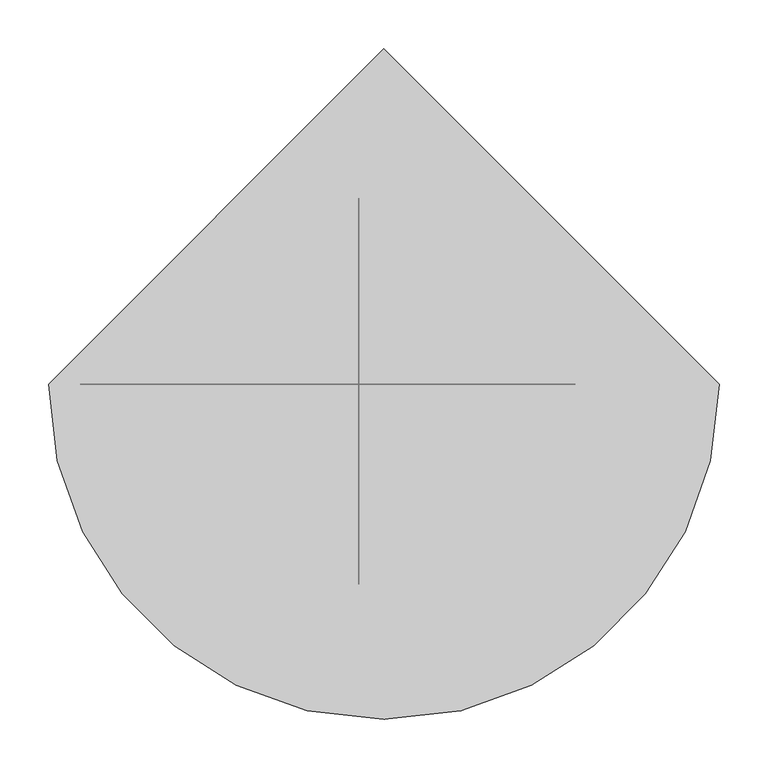
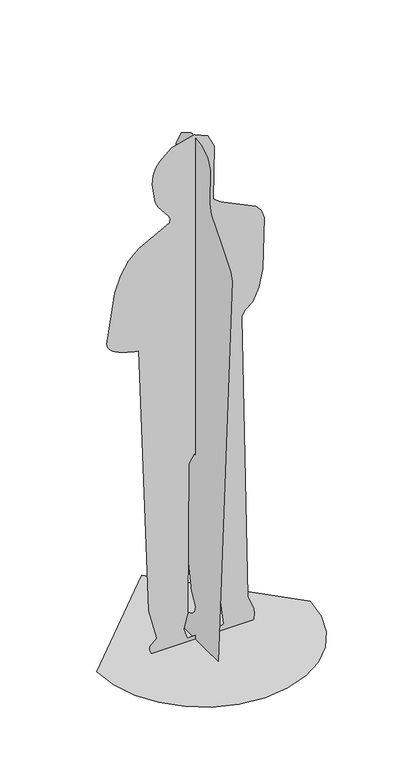
"""IFC4 building model written with IfcOpenShell, lengths in millimetres: proxy geometry, jay 23630 : jay 23630."""

import ifcopenshell
import ifcopenshell.guid

model = None  # the IFC model being written
_history = None  # IfcOwnerHistory: only IFC2X3 demands one
_inside = {}  # id of a spatial element -> (the spatial element, [elements in it])
_under = {}  # id of a project, library or spatial element -> (it, [spatial elements below it])
_declared = {}  # id of a project -> (the project, [libraries it declares])
_typed = {}  # id of a type object -> (the type object, [elements of that type])
_made_of = {}  # id of a material, layer set ... -> (it, [elements and type objects made of it])


def new_model(schema):
    """Start an empty IFC model of exactly this schema.

    Asked for "IFC4X3", IfcOpenShell would pick the latest addendum, in which some entities
    have other attributes; the version numbers below select the first issue.
    IFC2X3 requires an IfcOwnerHistory on every rooted entity: one is made here for all.
    """
    global model, _history
    if schema == "IFC4X3":
        model = ifcopenshell.file(schema_version=(4, 3, 0, 0))
    else:
        model = ifcopenshell.file(schema=schema)
    _inside.clear()
    _under.clear()
    _declared.clear()
    _typed.clear()
    _made_of.clear()
    _history = None
    if model.schema == "IFC2X3":
        org = make("IfcOrganization", Name="unknown")
        user = make(
            "IfcPersonAndOrganization",
            ThePerson=make("IfcPerson", FamilyName="unknown"),
            TheOrganization=org,
        )
        app = make(
            "IfcApplication",
            ApplicationDeveloper=org,
            Version="unknown",
            ApplicationFullName="unknown",
            ApplicationIdentifier="unknown",
        )
        _history = make(
            "IfcOwnerHistory",
            OwningUser=user,
            OwningApplication=app,
            ChangeAction="ADDED",
            CreationDate=0,
        )
    return model


def make(cls, **values):
    """One entity of the class cls with the attributes given. An attribute that is None is left unset."""
    return model.create_entity(
        cls, **{name: value for name, value in values.items() if value is not None}
    )


def rooted(cls, **values):
    """An entity with a GlobalId (a new one), such as an element, a storey or a relation."""
    return make(cls, GlobalId=ifcopenshell.guid.new(), OwnerHistory=_history, **values)


def si_unit(unit_type, name, prefix=None):
    """IfcSIUnit, for example si_unit("LENGTHUNIT", "METRE", prefix="MILLI")."""
    return make("IfcSIUnit", UnitType=unit_type, Prefix=prefix, Name=name)


def assignment(units):
    """IfcUnitAssignment: the units of a project."""
    return None if units is None else make("IfcUnitAssignment", Units=units)


def point(xyz):
    """IfcCartesianPoint."""
    return None if xyz is None else make("IfcCartesianPoint", Coordinates=xyz)


def direction(xyz):
    """IfcDirection."""
    return None if xyz is None else make("IfcDirection", DirectionRatios=xyz)


def frame(location, z_axis=None, x_axis=None):
    """IfcAxis2Placement3D, a coordinate frame: its origin and axes. An axis left out is left unset."""
    return make(
        "IfcAxis2Placement3D",
        Location=point(location),
        Axis=direction(z_axis),
        RefDirection=direction(x_axis),
    )


def origin():
    """The frame at (0, 0, 0) with its axes left unset."""
    return frame((0.0, 0.0, 0.0))


def place(relative_to, where):
    """IfcLocalPlacement: puts the frame where relative to a parent placement (None: the world)."""
    return make(
        "IfcLocalPlacement", PlacementRelTo=relative_to, RelativePlacement=where
    )


def context(
    kind, dimensions, precision=None, world=None, true_north=None, identifier=None
):
    """IfcGeometricRepresentationContext, for example the 3D "Model" context."""
    return make(
        "IfcGeometricRepresentationContext",
        ContextIdentifier=identifier,
        ContextType=kind,
        CoordinateSpaceDimension=dimensions,
        Precision=precision,
        WorldCoordinateSystem=world,
        TrueNorth=true_north,
    )


def project(units=None, contexts=None):
    """IfcProject with its units and contexts."""
    return rooted(
        "IfcProject",
        Name="project",
        RepresentationContexts=contexts,
        UnitsInContext=assignment(units),
    )


def spatial(cls, under=None, at=None, **own):
    """A site, building, storey or space (cls), placed at a placement, below another one or the project."""
    s = rooted(cls, ObjectPlacement=at, **own)
    if under is not None:
        _under.setdefault(under.id(), (under, []))[1].append(s)
    return s


def point_list(points):
    """IfcCartesianPointList2D or 3D."""
    cls = (
        "IfcCartesianPointList2D" if len(points[0]) == 2 else "IfcCartesianPointList3D"
    )
    return make(cls, CoordList=points)


def triangles(points, corners, closed=None, point_numbers=None):
    """IfcTriangulatedFaceSet: each triangle names its three corners, points numbered from 1."""
    return make(
        "IfcTriangulatedFaceSet",
        Coordinates=point_list(points),
        Closed=closed,
        CoordIndex=corners,
        PnIndex=point_numbers,
    )


def shape(context_of_items, identifier, shape_type, items):
    """IfcShapeRepresentation: the items that make up one representation, for example the "Body"."""
    return make(
        "IfcShapeRepresentation",
        ContextOfItems=context_of_items,
        RepresentationIdentifier=identifier,
        RepresentationType=shape_type,
        Items=items,
    )


def source(mapping_origin, context_of_items, identifier, shape_type, items):
    """IfcRepresentationMap: a shape defined once, which mapped items show again and again."""
    return make(
        "IfcRepresentationMap",
        MappingOrigin=mapping_origin,
        MappedRepresentation=shape(context_of_items, identifier, shape_type, items),
    )


def transform(
    local_origin,
    x_axis=None,
    y_axis=None,
    z_axis=None,
    scale=None,
    scale2=None,
    scale3=None,
    uniform=True,
):
    """IfcCartesianTransformationOperator3D, or its non-uniform kind. x_axis, y_axis, z_axis: its Axis1, 2, 3."""
    if uniform:
        return make(
            "IfcCartesianTransformationOperator3D",
            Axis1=direction(x_axis),
            Axis2=direction(y_axis),
            LocalOrigin=point(local_origin),
            Scale=scale,
            Axis3=direction(z_axis),
        )
    return make(
        "IfcCartesianTransformationOperator3DnonUniform",
        Axis1=direction(x_axis),
        Axis2=direction(y_axis),
        LocalOrigin=point(local_origin),
        Scale=scale,
        Axis3=direction(z_axis),
        Scale2=scale2,
        Scale3=scale3,
    )


def mapped(mapping_source, mapping_target):
    """IfcMappedItem: shows the shape of a source again, moved by a transform."""
    return make(
        "IfcMappedItem", MappingSource=mapping_source, MappingTarget=mapping_target
    )


def made_of(thing, what):
    """Note that an element or type object is made of a material, layer set ...; save() writes the relation."""
    if what is not None:
        _made_of.setdefault(what.id(), (what, []))[1].append(thing)
    return thing


def element(
    cls,
    number,
    at=None,
    inside=None,
    cuts=None,
    type_object=None,
    material=None,
    context=None,
    identifier="Body",
    shape_type=None,
    held_by="IfcProductDefinitionShape",
    body=None,
    shapes=None,
    **own,
):
    """One element of the class cls, such as IfcWall. Its Tag is "e" and its number.

    at: its placement. inside: the storey or other place that contains it. cuts: it is an
    opening in that element (IfcRelVoidsElement). A single representation is given by context,
    identifier, shape_type and body (its items); several are given by shapes. held_by: the class
    of the entity that holds the representations. save() writes the other relations.
    """
    e = rooted(cls, Tag="e%d" % number, ObjectPlacement=at, **own)
    if body is not None:
        shapes = [shape(context, identifier, shape_type, body)]
    if shapes is not None:
        e.Representation = make(held_by, Representations=shapes)
    if inside is not None:
        _inside.setdefault(inside.id(), (inside, []))[1].append(e)
    if cuts is not None:
        rooted(
            "IfcRelVoidsElement", RelatingBuildingElement=cuts, RelatedOpeningElement=e
        )
    if type_object is not None:
        _typed.setdefault(type_object.id(), (type_object, []))[1].append(e)
    return made_of(e, material)


def aggregate(whole, parts):
    """IfcRelAggregates: a whole, such as a stair, and the parts it consists of."""
    return rooted("IfcRelAggregates", RelatingObject=whole, RelatedObjects=parts)


def save(model, path):
    """Write the relations noted so far, then the file.

    IfcRelAggregates (storeys below a building ...), IfcRelContainedInSpatialStructure (elements
    in a storey), IfcRelDefinesByType, IfcRelAssociatesMaterial and IfcRelDeclares: one each for
    every whole, place, type object, material and project.
    """
    for whole, parts in _under.values():
        aggregate(whole, parts)
    for where, things in _inside.values():
        rooted(
            "IfcRelContainedInSpatialStructure",
            RelatedElements=things,
            RelatingStructure=where,
        )
    for kind, things in _typed.values():
        rooted("IfcRelDefinesByType", RelatedObjects=things, RelatingType=kind)
    for what, things in _made_of.values():
        rooted("IfcRelAssociatesMaterial", RelatedObjects=things, RelatingMaterial=what)
    for by, libraries in _declared.values():
        rooted("IfcRelDeclares", RelatingContext=by, RelatedDefinitions=libraries)
    model.write(path)


def entourage_8fcae429(model_context):
    return source(origin(), model_context, "Body", "Tessellation", [
        triangles([(-345.573129, 0.0, 0.0), (-336.4372767, -79.1825214, 0.0), (-310.4185887, -151.898995, 0.0), (-269.6002954, -216.0660267, 0.0), (-216.0660449, -269.6003499, 0.0), (-151.8989496, -310.4185161, 0.0), (-79.182476, -336.4372767, 0.0), (1.51e-05, -345.573129, 0.0), (79.1825214, -336.4373131, 0.0), (151.8990041, -310.4185887, 0.0), (216.0660449, -269.6002954, 0.0), (269.6004044, -216.0660449, 0.0), (310.4185524, -151.8989405, 0.0), (336.4372767, -79.1824669, 0.0), (345.573129, 3.02e-05, 0.0), (-4.53e-05, 345.573129, 0.0), (-25.78036, -206.1897945, 1348.8136002), (-25.78036, -197.5853052, 1374.9567719), (-25.78036, -143.9297776, 1440.4177471), (-25.78036, -88.0519655, 1504.3160271), (-25.78036, -79.0557305, 1537.7600613), (-25.78036, -83.3728362, 1655.4464825), (-25.78036, -70.0856975, 1687.5603653), (-25.78036, -36.8546772, 1709.6662834), (-25.78036, 23.8686285, 1717.8949963), (-25.78036, 79.9018998, 1684.0287495), (-25.78036, 106.2359483, 1634.1418236), (-25.78036, 109.3285375, 1576.3372124), (-25.78036, 95.6374309, 1518.7173283), (-25.78036, 71.6204603, 1469.3858917), (-25.78036, 43.7353573, 1436.4453152), (-25.78036, 18.439931, 1427.9987377), (-25.78036, 12.9047356, 1418.4000504), (-25.78036, 17.9030394, 1403.9002087), (-25.78036, 100.3158972, 1305.1847225), (-25.78036, 139.8422273, 1319.3011574), (-25.78036, 147.3154902, 1313.5241844), (-25.78036, 153.4761334, 1298.3650806), (-25.78036, 159.5450399, 1229.1756992), (-25.78036, 155.917754, 1209.0686417), (-25.78036, 148.709137, 1195.8695927), (-25.78036, 191.504717, 912.7641987), (-25.78036, 185.9813623, 822.2158739), (-25.78036, 168.0753332, 726.406097), (-25.78036, 163.1484355, 723.9989765), (-25.78036, 157.8330986, 724.045776), (-25.78036, 131.3723318, 737.6993757), (-25.78036, 21.417554, 149.8941936), (-25.78036, -1.3232615, 110.9245429), (-25.78036, 4.0590798, 90.9092221), (-25.78036, 18.2062061, 77.7815168), (-25.78036, 83.2378244, 46.7363279), (-25.78036, 102.4456182, 28.1713909), (-25.78036, 115.4189542, 0.0001939), (-25.78036, -127.8900044, 0.0001939), (-47.6681978, 5.01e-05, 607.394684), (-50.5685249, 7.96e-05, 98.4130518), (-63.1404637, 8.25e-05, 45.9886491), (-51.8472214, 8.45e-05, 12.1089164), (63.743988, 8.33e-05, 17.5652887), (66.5308818, 8.31e-05, 21.3655518), (-8.2278249, 5.05e-05, 609.0638409), (-29.2607276, 4.73e-05, 636.0603762), (-172.7832943, 8.44e-05, 13.4467537), (-173.6616201, 8.39e-05, 22.9478476), (-170.9381671, 8.35e-05, 29.5787746), (-154.6519156, 8.27e-05, 42.9999871), (-151.0159457, 8.23e-05, 48.9000085), (-176.6022473, 7.63e-05, 150.451091), (-208.3969635, 2.09e-05, 1050.4165524), (-216.4831887, 2.08e-05, 1051.9022175), (-226.3935031, 2.06e-05, 1053.8479563), (-237.6114049, 2.05e-05, 1056.3359585), (-249.6203194, 2.03e-05, 1059.4489225), (-261.9037993, 2.01e-05, 1063.2688929), (-273.9452518, 1.99e-05, 1067.8781319), (-285.228175, 1.97e-05, 1073.35912), (-292.7744804, 1.95e-05, 1078.0168299), (-299.4163715, 1.93e-05, 1083.228503), (-304.945558, 1.92e-05, 1089.0273497), (-309.1536223, 1.9e-05, 1095.4465799), (-311.8324196, 1.88e-05, 1102.5192587), (-312.7733505, 1.87e-05, 1110.2786688), (-311.7682157, 1.85e-05, 1118.7580204), (-286.8266966, 1.73e-05, 1275.1930939), (-267.1756069, 1.34e-05, 1328.1942192), (-240.945322, 8.5e-06, 1369.0343136), (-206.7917381, 3.8e-06, 1401.2005188), (-109.3374395, -1e-06, 1453.4599743), (-107.2218801, -2e-06, 1465.6289989), (-111.9356912, -3.4e-06, 1476.9063629), (-145.5691942, -7.6e-06, 1518.8280773), (-156.1162521, -8.3e-06, 1539.9788212), (-165.8142066, -1.06e-05, 1603.881752), (-162.2941272, -1.25e-05, 1633.2779228), (-153.7863434, -1.38e-05, 1656.3025349), (-141.886879, -1.48e-05, 1674.1116222), (-101.7987827, -1.66e-05, 1707.8037518), (-29.8635274, -1.51e-05, 1727.1999516), (13.7644623, -1.3e-05, 1708.5696934), (35.5195707, -1.05e-05, 1664.4861923), (32.4991723, -3.3e-06, 1485.0823174), (52.4866355, -2.3e-06, 1467.9128712), (169.1693616, 1.1e-06, 1411.612674), (187.957677, 2.2e-06, 1392.5309898), (197.4322985, 4e-06, 1363.4756413), (192.0197292, 1.43e-05, 1189.9500412), (178.7207045, 1.78e-05, 1132.0744314), (159.5661324, 2.03e-05, 1088.5580469), (134.4912548, 2.16e-05, 1068.0268147), (124.9300924, 2.55e-05, 1049.9808231), (143.8918166, 8.04e-05, 86.7553968), (162.7830327, 8.38e-05, 38.1705126), (165.3513534, 8.45e-05, 22.7356648), (163.2783513, 8.52e-05, 0.0004369), (-166.9538173, 8.52e-05, 0.0004369)], [[15, 16, 1], [14, 15, 1], [14, 1, 2], [13, 14, 2], [13, 2, 3], [13, 3, 4], [12, 13, 4], [11, 12, 4], [11, 4, 5], [11, 5, 6], [11, 6, 7], [11, 7, 8], [11, 8, 9], [11, 9, 10], [53, 54, 55], [52, 53, 55], [51, 52, 55], [50, 51, 55], [49, 50, 55], [48, 49, 55], [47, 48, 55], [47, 55, 17], [35, 36, 37], [35, 37, 38], [35, 38, 39], [43, 44, 45], [43, 45, 46], [43, 46, 47], [43, 47, 17], [42, 43, 17], [41, 42, 17], [41, 17, 18], [41, 18, 19], [40, 41, 19], [39, 40, 19], [35, 39, 19], [34, 35, 19], [33, 34, 19], [33, 19, 20], [32, 33, 20], [32, 20, 21], [31, 32, 21], [30, 31, 21], [29, 30, 21], [28, 29, 21], [27, 28, 21], [26, 27, 21], [25, 26, 21], [24, 25, 21], [24, 21, 22], [23, 24, 22], [114, 115, 116], [57, 58, 68], [57, 68, 69], [56, 57, 69], [56, 69, 70], [63, 56, 70], [68, 58, 59], [67, 68, 59], [66, 67, 59], [65, 66, 59], [64, 65, 59], [116, 64, 59], [99, 100, 101], [98, 99, 101], [97, 98, 101], [96, 97, 101], [95, 96, 101], [94, 95, 101], [93, 94, 101], [92, 93, 101], [91, 92, 101], [91, 101, 102], [90, 91, 102], [89, 90, 102], [89, 102, 103], [108, 109, 110], [104, 105, 106], [103, 104, 106], [89, 103, 106], [89, 106, 107], [89, 107, 108], [89, 108, 110], [88, 89, 110], [87, 88, 110], [86, 87, 110], [85, 86, 110], [84, 85, 110], [84, 110, 111], [83, 84, 111], [82, 83, 111], [81, 82, 111], [80, 81, 111], [79, 80, 111], [78, 79, 111], [77, 78, 111], [76, 77, 111], [75, 76, 111], [74, 75, 111], [73, 74, 111], [72, 73, 111], [71, 72, 111], [70, 71, 111], [63, 70, 111], [62, 63, 111], [61, 62, 111], [61, 111, 112], [61, 112, 113], [61, 113, 114], [60, 61, 114], [60, 114, 116], [60, 116, 59]], closed=False),
    ])


if __name__ == "__main__":
    model = new_model("IFC4")
    model_context = context("Model", 3, world=origin())
    ifc_project = project(units=[si_unit("LENGTHUNIT", "METRE", prefix="MILLI")], contexts=[model_context])
    site = spatial("IfcSite", under=ifc_project)
    building = spatial("IfcBuilding", under=site)
    placement = place(None, origin())
    entourage_shape = entourage_8fcae429(model_context)
    element("IfcBuildingElementProxy", 1, Name="jay 23630 : jay 23630", ObjectType="jay 23630 : jay 23630", at=placement, inside=building, context=model_context, shape_type="MappedRepresentation", body=[
        mapped(entourage_shape, transform((0.0, 0.0, 0.0), x_axis=(1.0, 0.0, 0.0), y_axis=(0.0, 1.0, 0.0), z_axis=(0.0, 0.0, 1.0))),
    ])
    save(model, "model.ifc")

# Revit data of these elements
# Type "jay 23630 : jay 23630"
#   built-in parameter 1005195 = "RPC-8-FWF3-6VPX-GP75-J"
#   Height = 0
